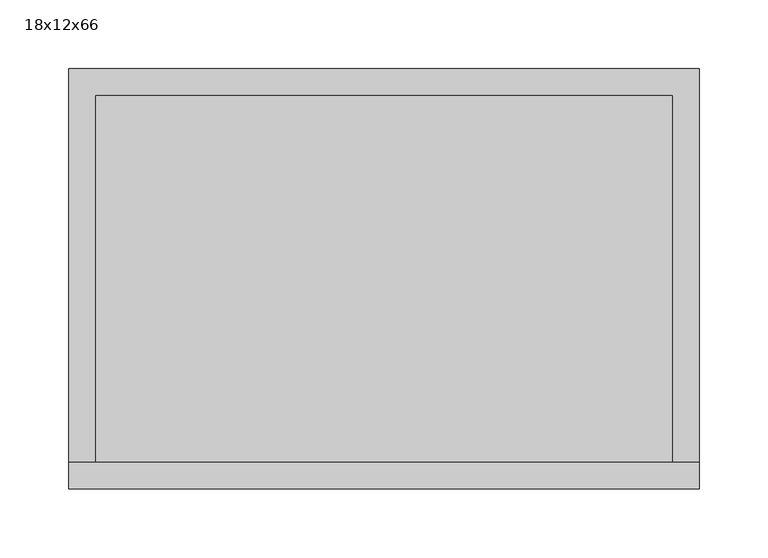
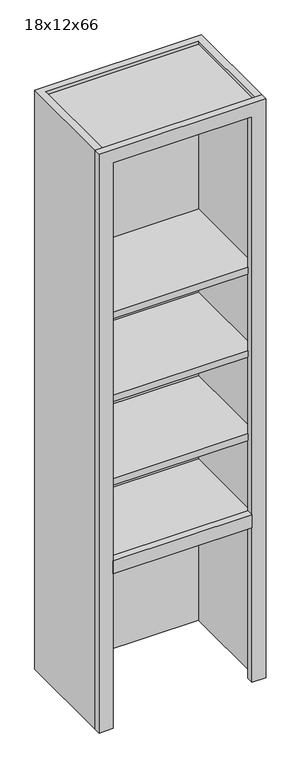
"""IFC4 building model written with IfcOpenShell, lengths in millimetres: furniture geometry, Bookcase-Merillat-Countertop : 18x12x66."""

from ifc_helpers import new_model, si_unit, frame, origin, place, context, project, spatial, polyline, outline, extrude, faceted_brep, source, transform, mapped, element, save


def furniture_18x12x66_d8155ed1(model_context):
    return source(origin(), model_context, "Body", "SolidModel", [
        extrude(outline(polyline([(-190.5, -133.35), (190.5, -133.35), (190.5, -152.4), (-190.5, -152.4), (-190.5, -133.35)])), frame((0.0, 0.0, 447.675), z_axis=(0.0, 0.0, 1.0), x_axis=(1.0, 0.0, 0.0)), (0.0, 0.0, 1.0), 38.1),
        extrude(outline(polyline([(-209.55, 133.35), (209.55, 133.35), (209.55, -133.35), (-209.55, -133.35), (-209.55, 133.35)])), frame((0.0, 0.0, 930.275), z_axis=(0.0, 0.0, 1.0), x_axis=(1.0, 0.0, 0.0)), (0.0, 0.0, 1.0), 19.3909952),
        extrude(outline(polyline([(-209.55, 133.35), (209.55, 133.35), (209.55, -133.35), (-209.55, -133.35), (-209.55, 133.35)])), frame((0.0, 0.0, 1171.2340048), z_axis=(0.0, 0.0, 1.0), x_axis=(1.0, 0.0, 0.0)), (0.0, 0.0, 1.0), 19.3909952),
        extrude(outline(polyline([(-209.55, 133.35), (209.55, 133.35), (209.55, -133.35), (-209.55, -133.35), (-209.55, 133.35)])), frame((0.0, 0.0, 688.8180074), z_axis=(0.0, 0.0, 1.0), x_axis=(1.0, 0.0, 0.0)), (0.0, 0.0, 1.0), 19.3909952),
        extrude(outline(polyline([(-209.55, 133.35), (209.55, 133.35), (209.55, -133.35), (-209.55, -133.35), (-209.55, 133.35)])), frame((0.0, 0.0, 447.675), z_axis=(0.0, 0.0, 1.0), x_axis=(1.0, 0.0, 0.0)), (0.0, 0.0, 1.0), 19.3909952),
        extrude(outline(polyline([(0.0, -228.6), (0.0, -190.5), (1638.3, -190.5), (1638.3, 190.5), (0.0, 190.5), (0.0, 228.6), (1676.4, 228.6), (1676.4, -228.6), (0.0, -228.6)])), frame((0.0, -152.4, 0.0), z_axis=(0.0, 1.0, 0.0), x_axis=(0.0, 0.0, 1.0)), (0.0, 0.0, 1.0), 19.05),
        faceted_brep([(-209.55, 133.35, 1667.1909423), (-209.55, -133.35, 1667.1909423), (209.55, -133.35, 1667.1909423), (209.55, 133.35, 1667.1909423), (-209.55, 133.35, 1676.4), (-209.55, -133.35, 1676.4), (209.55, -133.35, 1676.4), (209.55, 133.35, 1676.4), (-228.6, 152.4, 1676.4), (-228.6, -133.35, 1676.4), (228.6, -133.35, 1676.4), (228.6, 152.4, 1676.4), (-228.6, 152.4, 0.0), (228.6, 152.4, 0.0), (228.6, -133.35, 0.0), (209.55, -133.35, 0.0), (209.55, 133.35, 0.0), (-209.55, 133.35, 0.0), (-209.55, -133.35, 0.0), (-228.6, -133.35, 0.0), (-209.55, -133.35, 1657.0090048), (209.55, -133.35, 1657.0090048), (-209.55, 133.35, 1657.0090048), (209.55, 133.35, 1657.0090048)], [[[0, 1, 2, 3]], [[1, 0, 4, 5]], [[3, 2, 6, 7]], [[0, 3, 7, 4]], [[8, 9, 5, 4, 7, 6, 10, 11]], [[12, 13, 14, 15, 16, 17, 18, 19]], [[9, 8, 12, 19]], [[15, 14, 10, 6, 2, 1, 5, 9, 19, 18, 20, 21]], [[18, 17, 22, 20]], [[17, 16, 23, 22]], [[16, 15, 21, 23]], [[11, 10, 14, 13]], [[8, 11, 13, 12]], [[21, 20, 22, 23]]]),
    ])


if __name__ == "__main__":
    model = new_model("IFC4")
    model_context = context("Model", 3, world=origin())
    ifc_project = project(units=[si_unit("LENGTHUNIT", "METRE", prefix="MILLI")], contexts=[model_context])
    site = spatial("IfcSite", under=ifc_project)
    building = spatial("IfcBuilding", under=site)
    placement = place(None, origin())
    furniture_18x12x66_shape = furniture_18x12x66_d8155ed1(model_context)
    element("IfcFurniture", 1, ObjectType="Bookcase-Merillat-Countertop : 18x12x66", at=placement, inside=building, context=model_context, shape_type="MappedRepresentation", body=[
        mapped(furniture_18x12x66_shape, transform((0.0, 0.0, 0.0), x_axis=(1.0, 0.0, 0.0), y_axis=(0.0, 1.0, 0.0), z_axis=(0.0, 0.0, 1.0))),
    ])
    save(model, "model.ifc")

# Revit data of these elements
# Type "Bookcase-Merillat-Countertop : 18x12x66"
#   URL = "https://www.merillat.com/"
#   Product Page URL = "https://www.merillat.com/our-products/"
#   Product Documentation Link = "http://merillatbusiness.com/wp-content/uploads/2014/07/Merillat_Classic_Catalog.pdf"
#   Model = "BK1860"
#   Manufacturer = "Merillat"
#   Description = "Countertop Bookcase"
#   Construction Type = "Bookcase"
#   Assembly Code = "E2020200"
#   Width = 1' - 6"
#   Shelving Height = 0' - 9 1/2"
#   Height = 5' - 6"
#   Depth = 1' - 0"
#   Default Elevation = 2' - 6"
#   Cabinet Shell = 0' - 0 3/4"
#   COBie.Type = no
#   Number of Shelves = 5
#   Shelving Material = Wood - Merillat - Pecan(1)
#   Bookcase Material = Wood - Merillat - Pecan(1)
# Element 1 (IfcFurniture, "Bookcase-Merillat-Countertop : 18x12x66")
#   Materials on its faces: "Wood - Merillat - Pecan(1)"
# Materials
#   "Wood - Merillat - Pecan(1)": class "Wood", colour RGB 108 67 43, transparency 0, Cost = 0
